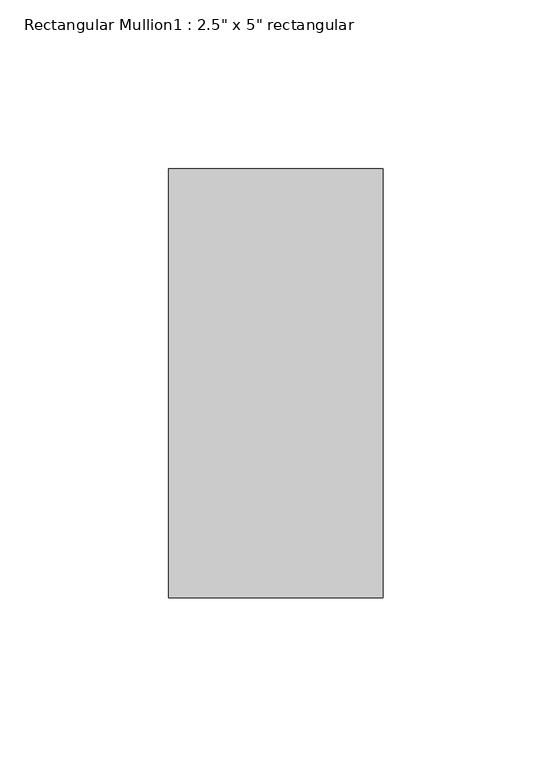
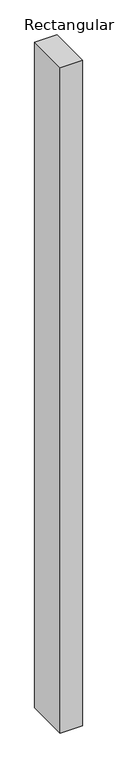
"""IFC4 building model written with IfcOpenShell, lengths in millimetres: member geometry."""

from ifc_helpers import new_model, si_unit, frame, origin, place, context, project, spatial, polyline, outline, extrude, source, transform, mapped, element, save


def member_3a2f4316(model_context):
    return source(origin(), model_context, "Body", "SweptSolid", [
        extrude(outline(polyline([(0.0, 63.5), (0.0, -63.5), (-63.5, -63.5), (-63.5, 63.5), (0.0, 63.5)])), frame((0.0, 0.0, -2021.4166667), z_axis=(0.0, 0.0, 1.0), x_axis=(1.0, 0.0, 0.0)), (0.0, 0.0, 1.0), 2021.4166667),
    ])


if __name__ == "__main__":
    model = new_model("IFC4")
    model_context = context("Model", 3, world=origin())
    ifc_project = project(units=[si_unit("LENGTHUNIT", "METRE", prefix="MILLI")], contexts=[model_context])
    site = spatial("IfcSite", under=ifc_project)
    building = spatial("IfcBuilding", under=site)
    placement = place(None, origin())
    member_shape = member_3a2f4316(model_context)
    element("IfcMember", 1, ObjectType="Rectangular Mullion1 : 2.5\" x 5\" rectangular", at=placement, inside=building, context=model_context, shape_type="MappedRepresentation", body=[
        mapped(member_shape, transform((0.0, 0.0, 0.0), x_axis=(1.0, 0.0, 0.0), y_axis=(0.0, 1.0, 0.0), z_axis=(0.0, 0.0, 1.0))),
    ])
    save(model, "model.ifc")

# Revit data of these elements
# Type "Rectangular Mullion1 : 2.5\" x 5\" rectangular"
#   built-in parameter 1007304 = 0.416667 (stored number, unit not read)
#   built-in parameter 1007301 = 0.104167 (stored number, unit not read)
#   built-in parameter 1007300 = 0.104167 (stored number, unit not read)
# Element 1 (IfcMember, "Rectangular Mullion1 : 2.5\" x 5\" rectangular")
#   Materials on its faces: "support-frame"
# Materials
#   "support-frame": class "Unassigned", colour RGB 233 233 233, transparency 0, Cost = 0
